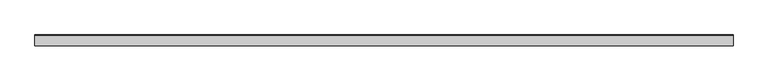
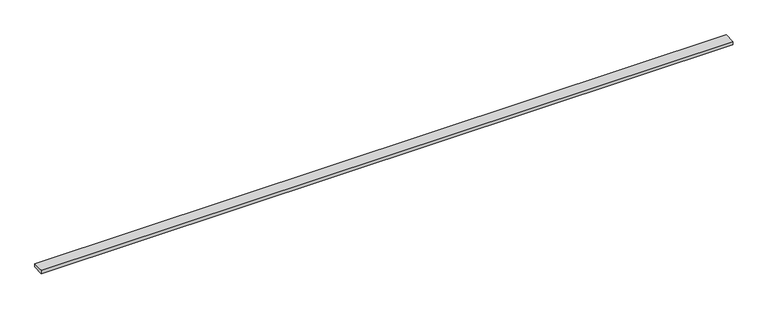
"""IFC4 building model written with IfcOpenShell, lengths in millimetres: proxy geometry, Inner panel:Inner panel:1:Inner panel:1 : Inner panel:Inner panel:300324:2:Inner panel:1:Inner panel:1 : Inner panel:Inner panel:300324:2 : Inner panel:Inner panel:1:Inner panel:1 : Inner panel:Inner panel:300324:300043:21 : Inner panel:Inner panel:1:Inner panel:1 : Inner panel:Inner panel:300324:2:Inner panel:1:Inner panel:1 : Inner panel:Inner panel:300324:2 : Inner panel:Inner panel:1:Inner panel:1 : Inner panel:Inner panel:300324:300043:308120."""

from ifc_helpers import new_model, si_unit, frame, origin, place, context, project, spatial, polyline, outline, extrude, source, transform, mapped, element, save


def generic_models_3e910e45(model_context):
    return source(origin(), model_context, "Body", "SweptSolid", [
        extrude(outline(polyline([(0.0, -75.8934963), (0.0, 0.0), (4876.8, 0.0), (4876.8, -75.8934963), (0.0, -75.8934963)])), frame((596182.8367242, -564971.654541, 8912.2317005), z_axis=(0.0, -0.04163054471214335, 0.9991330730923536), x_axis=(-1.0, 0.0, 0.0)), (0.0, 0.0, 1.0), 25.4),
    ])


if __name__ == "__main__":
    model = new_model("IFC4")
    model_context = context("Model", 3, world=origin())
    ifc_project = project(units=[si_unit("LENGTHUNIT", "METRE", prefix="MILLI")], contexts=[model_context])
    site = spatial("IfcSite", under=ifc_project)
    building = spatial("IfcBuilding", under=site)
    placement = place(None, origin())
    generic_models_shape = generic_models_3e910e45(model_context)
    element("IfcBuildingElementProxy", 1, Name="Inner panel:Inner panel:1:Inner panel:1 : Inner panel:Inner panel:300324:2:Inner panel:1:Inner panel:1 : Inner panel:Inner panel:300324:2 : Inner panel:Inner panel:1:Inner panel:1 : Inner panel:Inner panel:300324:300043:21 : Inner panel:Inner panel:1:Inner panel:1 : Inner panel:Inner panel:300324:2:Inner panel:1:Inner panel:1 : Inner panel:Inner panel:300324:2 : Inner panel:Inner panel:1:Inner panel:1 : Inner panel:Inner panel:300324:300043:308120", ObjectType="Inner panel:Inner panel:1:Inner panel:1 : Inner panel:Inner panel:300324:2:Inner panel:1:Inner panel:1 : Inner panel:Inner panel:300324:2 : Inner panel:Inner panel:1:Inner panel:1 : Inner panel:Inner panel:300324:300043:21 : Inner panel:Inner panel:1:Inner panel:1 : Inner panel:Inner panel:300324:2:Inner panel:1:Inner panel:1 : Inner panel:Inner panel:300324:2 : Inner panel:Inner panel:1:Inner panel:1 : Inner panel:Inner panel:300324:300043:308120", at=placement, inside=building, context=model_context, shape_type="MappedRepresentation", body=[
        mapped(generic_models_shape, transform((0.0, 0.0, 0.0), x_axis=(1.0, 0.0, 0.0), y_axis=(0.0, 1.0, 0.0), z_axis=(0.0, 0.0, 1.0))),
    ])
    save(model, "model.ifc")

# Revit data of these elements
# Type "Inner panel:Inner panel:1:Inner panel:1 : Inner panel:Inner panel:300324:2:Inner panel:1:Inner panel:1 : Inner panel:Inner panel:300324:2 : Inner panel:Inner panel:1:Inner panel:1 : Inner panel:Inner panel:300324:300043:21 : Inner panel:Inner panel:1:Inner panel:1 : Inner panel:Inner panel:300324:2:Inner panel:1:Inner panel:1 : Inner panel:Inner panel:300324:2 : Inner panel:Inner panel:1:Inner panel:1 : Inner panel:Inner panel:300324:300043:308120"
#   NameOverride = "Inner panel:Inner panel:1:Inner panel:1 : Inner panel:Inner panel:300324:2:Inner panel:1:Inner panel:1 : Inner panel:Inner panel:300324:2 : Inner panel:Inner panel:1:Inner panel:1 : Inner panel:Inner panel:300324:300043:308120"
#   ObjectTypeOverride = "Inner panel:1:Inner panel:1 : Inner panel:Inner panel:300324:2 : Inner panel:Inner panel:1:Inner panel:1 : Inner panel:Inner panel:300324:300043"
#   Reference = "Inner panel"
#   Tag = "308120"
# Element 1 (IfcBuildingElementProxy, "Inner panel:Inner panel:1:Inner panel:1 : Inner panel:Inner panel:300324:2:Inner panel:1:Inner panel:1 : Inner panel:Inner panel:300324:2 : Inner panel:Inner panel:1:Inner panel:1 : Inner panel:Inner panel:300324:300043:21 : Inner panel:Inner panel:1:Inner panel:1 : Inner panel:Inner panel:300324:2:Inner panel:1:Inner panel:1 : Inner panel:Inner panel:300324:2 : Inner panel:Inner panel:1:Inner panel:1 : Inner panel:Inner panel:300324:300043:308120")
#   Materials on its faces: "1\" THERMAL SPACER @ PURLIN"
# Materials
#   "1\" THERMAL SPACER @ PURLIN": class "Unassigned", colour RGB 205 188 106, transparency 0, Cost = 0
